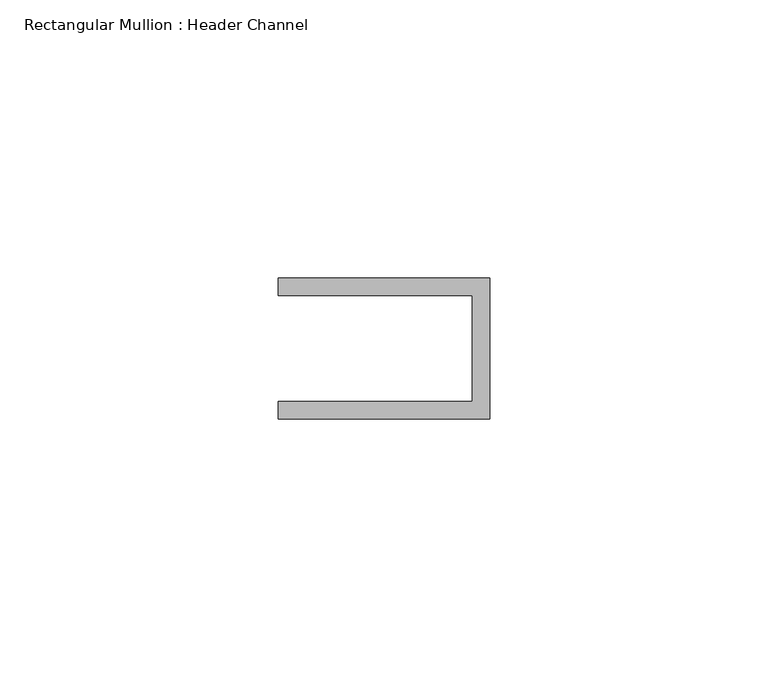
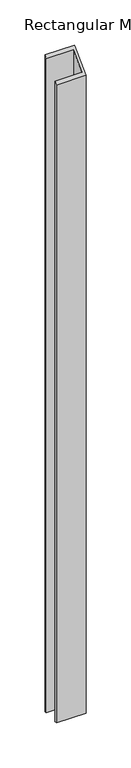
"""IFC4 building model written with IfcOpenShell, lengths in millimetres: member geometry, Rectangular Mullion : Header Channel."""

from ifc_helpers import new_model, si_unit, origin, place, context, project, spatial, faceted_brep, source, transform, mapped, element, save


def rectangular_mullion_header_channel_1899376f(model_context):
    return source(origin(), model_context, "Body", "Brep", [
        faceted_brep([(0.0, 12.7, -876.6175002), (0.0, -12.7, -876.6175002), (-38.1, -12.7, -876.6175002), (-38.1, -9.525, -876.6175002), (-3.175, -9.525, -876.6175002), (-3.175, 9.525, -876.6175002), (-38.1, 9.525, -876.6175002), (-38.1, 12.7, -876.6175002), (-38.1, 12.7, 12.7), (0.0, 12.7, 12.7), (-38.1, 9.525, 9.525), (-3.175, 9.525, 9.525), (-3.175, -9.525, -9.525), (-38.1, -9.525, -9.525), (-38.1, -12.7, -12.7), (0.0, -12.7, -12.7)], [[[0, 1, 2, 3, 4, 5, 6, 7]], [[8, 9, 0, 7]], [[10, 8, 7, 6]], [[11, 10, 6, 5]], [[12, 11, 5, 4]], [[13, 12, 4, 3]], [[14, 13, 3, 2]], [[15, 14, 2, 1]], [[9, 15, 1, 0]], [[9, 8, 10, 11, 12, 13, 14, 15]]]),
    ])


if __name__ == "__main__":
    model = new_model("IFC4")
    model_context = context("Model", 3, world=origin())
    ifc_project = project(units=[si_unit("LENGTHUNIT", "METRE", prefix="MILLI")], contexts=[model_context])
    site = spatial("IfcSite", under=ifc_project)
    building = spatial("IfcBuilding", under=site)
    placement = place(None, origin())
    rectangular_mullion_header_channel_shape = rectangular_mullion_header_channel_1899376f(model_context)
    element("IfcMember", 1, ObjectType="Rectangular Mullion : Header Channel", at=placement, inside=building, context=model_context, shape_type="MappedRepresentation", body=[
        mapped(rectangular_mullion_header_channel_shape, transform((0.0, 0.0, 0.0), x_axis=(1.0, 0.0, 0.0), y_axis=(0.0, 1.0, 0.0), z_axis=(0.0, 0.0, 1.0))),
    ])
    save(model, "model.ifc")

# Revit data of these elements
# Type "Rectangular Mullion : Header Channel"
#   built-in parameter 1007322 = 0.0833333 (stored number, unit not read)
#   built-in parameter 1007321 = -0.03125 (stored number, unit not read)
#   built-in parameter 1007320 = 0.0416667 (stored number, unit not read)
# Element 1 (IfcMember, "Rectangular Mullion : Header Channel")
#   Materials on its faces: "ALUM"
# Materials
#   "ALUM": class "Generic", colour RGB 157 157 157, transparency 0, Cost = 0
